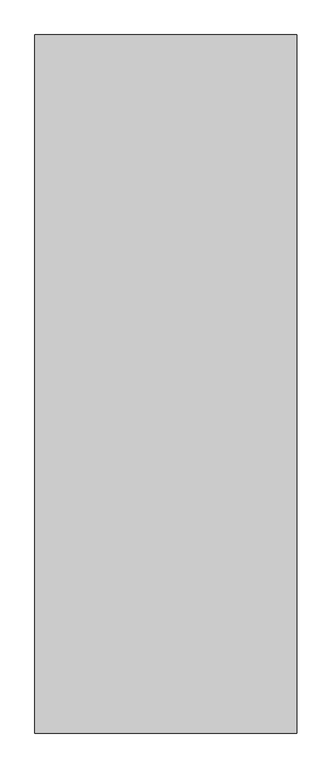
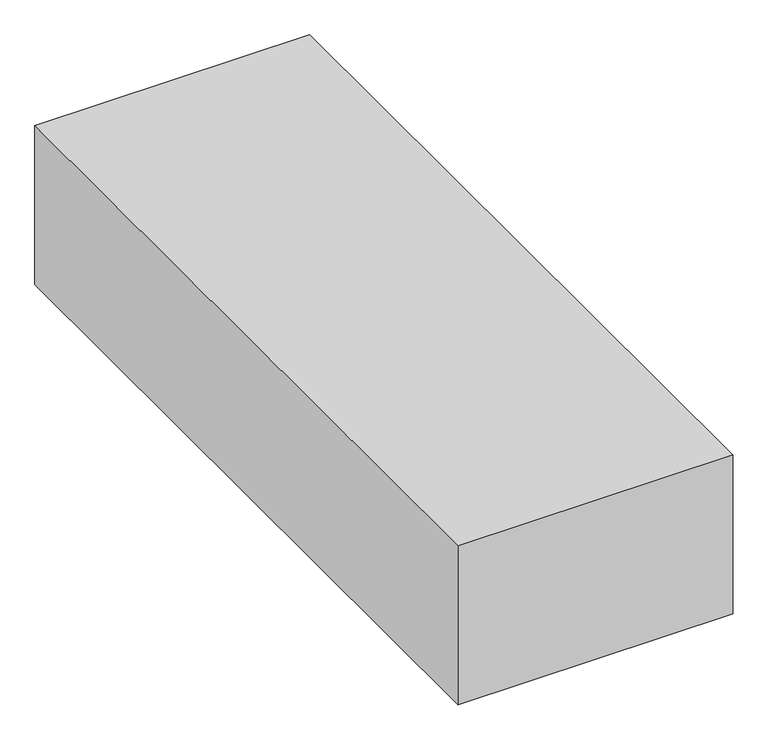
"""IFC4 building model written with IfcOpenShell, lengths in millimetres: proxy geometry, Space Planning Box_hec : Space Planning Box_hec."""

import ifcopenshell
import ifcopenshell.guid

model = None  # the IFC model being written
_history = None  # IfcOwnerHistory: only IFC2X3 demands one
_inside = {}  # id of a spatial element -> (the spatial element, [elements in it])
_under = {}  # id of a project, library or spatial element -> (it, [spatial elements below it])
_declared = {}  # id of a project -> (the project, [libraries it declares])
_typed = {}  # id of a type object -> (the type object, [elements of that type])
_made_of = {}  # id of a material, layer set ... -> (it, [elements and type objects made of it])


def new_model(schema):
    """Start an empty IFC model of exactly this schema.

    Asked for "IFC4X3", IfcOpenShell would pick the latest addendum, in which some entities
    have other attributes; the version numbers below select the first issue.
    IFC2X3 requires an IfcOwnerHistory on every rooted entity: one is made here for all.
    """
    global model, _history
    if schema == "IFC4X3":
        model = ifcopenshell.file(schema_version=(4, 3, 0, 0))
    else:
        model = ifcopenshell.file(schema=schema)
    _inside.clear()
    _under.clear()
    _declared.clear()
    _typed.clear()
    _made_of.clear()
    _history = None
    if model.schema == "IFC2X3":
        org = make("IfcOrganization", Name="unknown")
        user = make(
            "IfcPersonAndOrganization",
            ThePerson=make("IfcPerson", FamilyName="unknown"),
            TheOrganization=org,
        )
        app = make(
            "IfcApplication",
            ApplicationDeveloper=org,
            Version="unknown",
            ApplicationFullName="unknown",
            ApplicationIdentifier="unknown",
        )
        _history = make(
            "IfcOwnerHistory",
            OwningUser=user,
            OwningApplication=app,
            ChangeAction="ADDED",
            CreationDate=0,
        )
    return model


def make(cls, **values):
    """One entity of the class cls with the attributes given. An attribute that is None is left unset."""
    return model.create_entity(
        cls, **{name: value for name, value in values.items() if value is not None}
    )


def rooted(cls, **values):
    """An entity with a GlobalId (a new one), such as an element, a storey or a relation."""
    return make(cls, GlobalId=ifcopenshell.guid.new(), OwnerHistory=_history, **values)


def si_unit(unit_type, name, prefix=None):
    """IfcSIUnit, for example si_unit("LENGTHUNIT", "METRE", prefix="MILLI")."""
    return make("IfcSIUnit", UnitType=unit_type, Prefix=prefix, Name=name)


def assignment(units):
    """IfcUnitAssignment: the units of a project."""
    return None if units is None else make("IfcUnitAssignment", Units=units)


def point(xyz):
    """IfcCartesianPoint."""
    return None if xyz is None else make("IfcCartesianPoint", Coordinates=xyz)


def direction(xyz):
    """IfcDirection."""
    return None if xyz is None else make("IfcDirection", DirectionRatios=xyz)


def frame(location, z_axis=None, x_axis=None):
    """IfcAxis2Placement3D, a coordinate frame: its origin and axes. An axis left out is left unset."""
    return make(
        "IfcAxis2Placement3D",
        Location=point(location),
        Axis=direction(z_axis),
        RefDirection=direction(x_axis),
    )


def origin():
    """The frame at (0, 0, 0) with its axes left unset."""
    return frame((0.0, 0.0, 0.0))


def origin_with_axes():
    """The frame at (0, 0, 0) with the z axis (0, 0, 1) and the x axis (1, 0, 0) written out."""
    return frame((0.0, 0.0, 0.0), z_axis=(0.0, 0.0, 1.0), x_axis=(1.0, 0.0, 0.0))


def place(relative_to, where):
    """IfcLocalPlacement: puts the frame where relative to a parent placement (None: the world)."""
    return make(
        "IfcLocalPlacement", PlacementRelTo=relative_to, RelativePlacement=where
    )


def context(
    kind, dimensions, precision=None, world=None, true_north=None, identifier=None
):
    """IfcGeometricRepresentationContext, for example the 3D "Model" context."""
    return make(
        "IfcGeometricRepresentationContext",
        ContextIdentifier=identifier,
        ContextType=kind,
        CoordinateSpaceDimension=dimensions,
        Precision=precision,
        WorldCoordinateSystem=world,
        TrueNorth=true_north,
    )


def project(units=None, contexts=None):
    """IfcProject with its units and contexts."""
    return rooted(
        "IfcProject",
        Name="project",
        RepresentationContexts=contexts,
        UnitsInContext=assignment(units),
    )


def spatial(cls, under=None, at=None, **own):
    """A site, building, storey or space (cls), placed at a placement, below another one or the project."""
    s = rooted(cls, ObjectPlacement=at, **own)
    if under is not None:
        _under.setdefault(under.id(), (under, []))[1].append(s)
    return s


def polyline(points):
    """IfcPolyline through the points."""
    return make("IfcPolyline", Points=[point(p) for p in points])


def outline(outer, holes=None, kind="AREA"):
    """IfcArbitraryClosedProfileDef: a profile drawn as a closed curve; with holes, ...WithVoids."""
    if holes is None:
        return make("IfcArbitraryClosedProfileDef", ProfileType=kind, OuterCurve=outer)
    return make(
        "IfcArbitraryProfileDefWithVoids",
        ProfileType=kind,
        OuterCurve=outer,
        InnerCurves=holes,
    )


def extrude(swept, where, along, depth):
    """IfcExtrudedAreaSolid: the profile swept, set in the frame where, extruded along a direction by depth."""
    return make(
        "IfcExtrudedAreaSolid",
        SweptArea=swept,
        Position=where,
        ExtrudedDirection=direction(along),
        Depth=depth,
    )


def shape(context_of_items, identifier, shape_type, items):
    """IfcShapeRepresentation: the items that make up one representation, for example the "Body"."""
    return make(
        "IfcShapeRepresentation",
        ContextOfItems=context_of_items,
        RepresentationIdentifier=identifier,
        RepresentationType=shape_type,
        Items=items,
    )


def source(mapping_origin, context_of_items, identifier, shape_type, items):
    """IfcRepresentationMap: a shape defined once, which mapped items show again and again."""
    return make(
        "IfcRepresentationMap",
        MappingOrigin=mapping_origin,
        MappedRepresentation=shape(context_of_items, identifier, shape_type, items),
    )


def transform(
    local_origin,
    x_axis=None,
    y_axis=None,
    z_axis=None,
    scale=None,
    scale2=None,
    scale3=None,
    uniform=True,
):
    """IfcCartesianTransformationOperator3D, or its non-uniform kind. x_axis, y_axis, z_axis: its Axis1, 2, 3."""
    if uniform:
        return make(
            "IfcCartesianTransformationOperator3D",
            Axis1=direction(x_axis),
            Axis2=direction(y_axis),
            LocalOrigin=point(local_origin),
            Scale=scale,
            Axis3=direction(z_axis),
        )
    return make(
        "IfcCartesianTransformationOperator3DnonUniform",
        Axis1=direction(x_axis),
        Axis2=direction(y_axis),
        LocalOrigin=point(local_origin),
        Scale=scale,
        Axis3=direction(z_axis),
        Scale2=scale2,
        Scale3=scale3,
    )


def mapped(mapping_source, mapping_target):
    """IfcMappedItem: shows the shape of a source again, moved by a transform."""
    return make(
        "IfcMappedItem", MappingSource=mapping_source, MappingTarget=mapping_target
    )


def made_of(thing, what):
    """Note that an element or type object is made of a material, layer set ...; save() writes the relation."""
    if what is not None:
        _made_of.setdefault(what.id(), (what, []))[1].append(thing)
    return thing


def element(
    cls,
    number,
    at=None,
    inside=None,
    cuts=None,
    type_object=None,
    material=None,
    context=None,
    identifier="Body",
    shape_type=None,
    held_by="IfcProductDefinitionShape",
    body=None,
    shapes=None,
    **own,
):
    """One element of the class cls, such as IfcWall. Its Tag is "e" and its number.

    at: its placement. inside: the storey or other place that contains it. cuts: it is an
    opening in that element (IfcRelVoidsElement). A single representation is given by context,
    identifier, shape_type and body (its items); several are given by shapes. held_by: the class
    of the entity that holds the representations. save() writes the other relations.
    """
    e = rooted(cls, Tag="e%d" % number, ObjectPlacement=at, **own)
    if body is not None:
        shapes = [shape(context, identifier, shape_type, body)]
    if shapes is not None:
        e.Representation = make(held_by, Representations=shapes)
    if inside is not None:
        _inside.setdefault(inside.id(), (inside, []))[1].append(e)
    if cuts is not None:
        rooted(
            "IfcRelVoidsElement", RelatingBuildingElement=cuts, RelatedOpeningElement=e
        )
    if type_object is not None:
        _typed.setdefault(type_object.id(), (type_object, []))[1].append(e)
    return made_of(e, material)


def aggregate(whole, parts):
    """IfcRelAggregates: a whole, such as a stair, and the parts it consists of."""
    return rooted("IfcRelAggregates", RelatingObject=whole, RelatedObjects=parts)


def save(model, path):
    """Write the relations noted so far, then the file.

    IfcRelAggregates (storeys below a building ...), IfcRelContainedInSpatialStructure (elements
    in a storey), IfcRelDefinesByType, IfcRelAssociatesMaterial and IfcRelDeclares: one each for
    every whole, place, type object, material and project.
    """
    for whole, parts in _under.values():
        aggregate(whole, parts)
    for where, things in _inside.values():
        rooted(
            "IfcRelContainedInSpatialStructure",
            RelatedElements=things,
            RelatingStructure=where,
        )
    for kind, things in _typed.values():
        rooted("IfcRelDefinesByType", RelatedObjects=things, RelatingType=kind)
    for what, things in _made_of.values():
        rooted("IfcRelAssociatesMaterial", RelatedObjects=things, RelatingMaterial=what)
    for by, libraries in _declared.values():
        rooted("IfcRelDeclares", RelatingContext=by, RelatedDefinitions=libraries)
    model.write(path)


def generic_models_7ea3b148(model_context):
    return source(origin(), model_context, "Body", "SweptSolid", [
        extrude(outline(polyline([(4500.0, 12000.0), (4500.0, -12000.0), (-4500.0, -12000.0), (-4500.0, 12000.0), (4500.0, 12000.0)])), origin_with_axes(), (0.0, 0.0, 1.0), 5500.0),
    ])


if __name__ == "__main__":
    model = new_model("IFC4")
    model_context = context("Model", 3, world=origin())
    ifc_project = project(units=[si_unit("LENGTHUNIT", "METRE", prefix="MILLI")], contexts=[model_context])
    site = spatial("IfcSite", under=ifc_project)
    building = spatial("IfcBuilding", under=site)
    placement = place(None, origin())
    generic_models_shape = generic_models_7ea3b148(model_context)
    element("IfcBuildingElementProxy", 1, Name="Space Planning Box_hec : Space Planning Box_hec", ObjectType="Space Planning Box_hec : Space Planning Box_hec", at=placement, inside=building, context=model_context, shape_type="MappedRepresentation", body=[
        mapped(generic_models_shape, transform((0.0, 0.0, 0.0), x_axis=(1.0, 0.0, 0.0), y_axis=(0.0, 1.0, 0.0), z_axis=(0.0, 0.0, 1.0))),
    ])
    save(model, "model.ifc")

# Revit data of these elements
# Type "Space Planning Box_hec : Space Planning Box_hec"
#   Type Comments = "..."
#   Room Name [instance default] = "?"
#   Interior Finish [instance default] = ""
#   Exterior Finish [instance default] = ""
#   Department [instance default] = ""
#   Assembly Code = "..."
#   ceiling height [instance default] = 0
#   Width [instance default] = 1524 mm
#   Program Area [instance default] = 0.00 m²
#   Length [instance default] = 1524 mm
#   Height [instance default] = 1524 mm
#   Area [instance default] = 2.32258 m²
#   Fill Color [instance default] = Cyan
#   Default Elevation = 0
# Element 1 (IfcBuildingElementProxy, "Space Planning Box_hec : Space Planning Box_hec")
#   Room Name = "Central Control Room"
#   Exterior Finish = "N/A..N/A,,EW1..N/A..N/A"
#   Department = "CI"
#   Width = 9000 mm
#   Program Area = 216.00 m²
#   Length = 24000 mm
#   Height = 5500 mm
#   Area = 216.00 m²
#   Fill Color = Yellow
#   Materials on its faces: "Yellow"
# Materials
#   "Cyan": class "Generic", colour RGB 0 255 255, transparency 0.2, Cost = 0
#   "Yellow": class "Generic", colour RGB 255 255 0, transparency 0.2, Cost = 0
